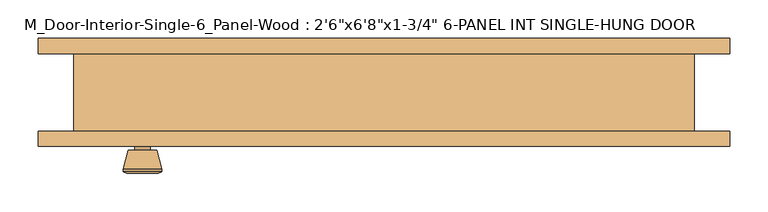
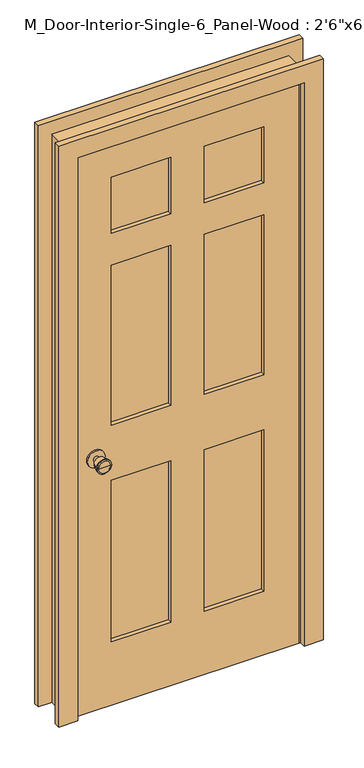
"""IFC4 building model written with IfcOpenShell, lengths in millimetres: door geometry."""

from ifc_helpers import new_model, si_unit, point, frame, frame_2d, origin, place, context, project, spatial, polyline, circle_curve, trimmed, segment, composite_curve, outline, extrude, faceted_brep, source, transform, mapped, element, save
from ifc_brep_helpers import plane_surface, cylinder_surface, revolved_surface, advanced_brep


def door_8e0f4bcc(model_context):
    return source(origin(), model_context, "Body", "SolidModel", [
        advanced_brep(
        [(-316.0, 2.825, 914.4), (-326.0, 2.825, 914.4), (-306.0, 2.825, 914.4), (-295.5241324, 51.825, 914.4), (-336.4758676, 51.825, 914.4), (-316.0, 51.825, 914.4), (-291.0, 49.9971319, 914.4), (-341.0, 49.9971319, 914.4), (-291.0, 46.5334537, 914.4), (-341.0, 46.5334537, 914.4), (-297.363764, 21.825, 914.4), (-334.636236, 21.825, 914.4), (-306.0, 21.825, 914.4), (-326.0, 21.825, 914.4)],
        [
            (0, 1),
            (1, 2, circle_curve(frame((-316.0, 2.825, 914.4), z_axis=(0.0, -1.0, 0.0), x_axis=(-1.0, 0.0, 0.0)), 10.0)),
            (2, 0),
            (2, 1, circle_curve(frame((-316.0, 2.825, 914.4), z_axis=(0.0, -1.0, 0.0), x_axis=(-1.0, 0.0, 0.0)), 10.0)),
            (3, 4, circle_curve(frame((-316.0, 51.825, 914.4), z_axis=(0.0, 1.0, 0.0), x_axis=(-1.0, 0.0, 0.0)), 20.4758676)),
            (4, 5),
            (5, 3),
            (4, 3, circle_curve(frame((-316.0, 51.825, 914.4), z_axis=(0.0, 1.0, 0.0), x_axis=(-1.0, 0.0, 0.0)), 20.4758676)),
            (6, 7, circle_curve(frame((-316.0, 49.9971319, 914.4), z_axis=(0.0, 1.0, 0.0), x_axis=(-1.0, 0.0, 0.0)), 25.0)),
            (7, 4),
            (3, 6),
            (7, 6, circle_curve(frame((-316.0, 49.9971319, 914.4), z_axis=(0.0, 1.0, 0.0), x_axis=(-1.0, 0.0, 0.0)), 25.0)),
            (8, 9, circle_curve(frame((-316.0, 46.5334537, 914.4), z_axis=(0.0, 1.0, 0.0), x_axis=(-1.0, 0.0, 0.0)), 25.0)),
            (9, 7),
            (6, 8),
            (9, 8, circle_curve(frame((-316.0, 46.5334537, 914.4), z_axis=(0.0, 1.0, 0.0), x_axis=(-1.0, 0.0, 0.0)), 25.0)),
            (10, 11, circle_curve(frame((-316.0, 21.825, 914.4), z_axis=(0.0, 1.0, 0.0), x_axis=(-1.0, 0.0, 0.0)), 18.636236)),
            (11, 9),
            (8, 10),
            (11, 10, circle_curve(frame((-316.0, 21.825, 914.4), z_axis=(0.0, 1.0, 0.0), x_axis=(-1.0, 0.0, 0.0)), 18.636236)),
            (12, 13, circle_curve(frame((-316.0, 21.825, 914.4), z_axis=(0.0, 1.0, 0.0), x_axis=(-1.0, 0.0, 0.0)), 10.0)),
            (13, 11),
            (10, 12),
            (13, 12, circle_curve(frame((-316.0, 21.825, 914.4), z_axis=(0.0, 1.0, 0.0), x_axis=(-1.0, 0.0, 0.0)), 10.0)),
            (1, 13),
            (12, 2),
        ],
        [
            plane_surface(frame((-316.0, 2.825, 914.4), z_axis=(0.0, -1.0, 0.0), x_axis=(-1.0, 0.0, 0.0))),
            plane_surface(frame((-316.0, 51.825, 914.4), z_axis=(0.0, 1.0, 0.0), x_axis=(-1.0, 0.0, 0.0))),
            revolved_surface(polyline([(-336.4758676, 51.825, 914.4), (-341.0, 49.9971319, 914.4)]), (-316.0, 2.825, 914.4), (0.0, -1.0, 0.0)),
            cylinder_surface(frame((-316.0, 2.825, 914.4), z_axis=(0.0, -1.0, 0.0), x_axis=(-1.0, 0.0, 0.0)), 25.0),
            revolved_surface(polyline([(-341.0, 46.5334537, 914.4), (-334.636236, 21.825, 914.4)]), (-316.0, 2.825, 914.4), (0.0, -1.0, 0.0)),
            plane_surface(frame((-316.0, 21.825, 914.4), z_axis=(0.0, -1.0, 0.0), x_axis=(-1.0, 0.0, 0.0))),
            cylinder_surface(frame((-316.0, 2.825, 914.4), z_axis=(0.0, -1.0, 0.0), x_axis=(-1.0, 0.0, 0.0)), 10.0),
        ],
        [
            (0, [[1, 2, 3]]),
            (0, [[-3, 4, -1]]),
            (1, [[5, 6, 7]]),
            (1, [[8, -7, -6]]),
            (2, [[9, 10, -5, 11]]),
            (2, [[12, -11, -8, -10]]),
            (3, [[13, 14, -9, 15]]),
            (3, [[16, -15, -12, -14]]),
            (4, [[17, 18, -13, 19]]),
            (4, [[20, -19, -16, -18]]),
            (5, [[21, 22, -17, 23]]),
            (5, [[24, -23, -20, -22]]),
            (6, [[-2, 25, -21, 26]]),
            (6, [[-4, -26, -24, -25]]),
        ],
    ),
        extrude(outline(composite_curve([segment(trimmed(circle_curve(frame_2d((914.4, -316.0)), 30.0), [point((914.4, -346.0))], [point((914.4, -286.0))], False, "CARTESIAN"), True, "CONTINUOUS"), segment(trimmed(circle_curve(frame_2d((914.4, -316.0)), 30.0), [point((914.4, -286.0))], [point((914.4, -346.0))], False, "CARTESIAN"), True, "CONTINUOUS")], self_intersect=False)), frame((0.0, -3.175, 0.0), z_axis=(0.0, 1.0, 0.0), x_axis=(0.0, 0.0, 1.0)), (0.0, 0.0, 1.0), 6.0),
        advanced_brep(
        [(-316.0, -53.625, 914.4), (-306.0, -53.625, 914.4), (-326.0, -53.625, 914.4), (-295.5241324, -102.625, 914.4), (-316.0, -102.625, 914.4), (-336.4758676, -102.625, 914.4), (-291.0, -100.7971319, 914.4), (-341.0, -100.7971319, 914.4), (-291.0, -97.3334537, 914.4), (-341.0, -97.3334537, 914.4), (-297.363764, -72.625, 914.4), (-334.636236, -72.625, 914.4), (-306.0, -72.625, 914.4), (-326.0, -72.625, 914.4)],
        [
            (0, 1),
            (1, 2, circle_curve(frame((-316.0, -53.625, 914.4), z_axis=(0.0, 1.0, 0.0), x_axis=(-1.0, 0.0, 0.0)), 10.0)),
            (2, 0),
            (2, 1, circle_curve(frame((-316.0, -53.625, 914.4), z_axis=(0.0, 1.0, 0.0), x_axis=(-1.0, 0.0, 0.0)), 10.0)),
            (3, 4),
            (4, 5),
            (5, 3, circle_curve(frame((-316.0, -102.625, 914.4), z_axis=(0.0, -1.0, 0.0), x_axis=(-1.0, 0.0, 0.0)), 20.4758676)),
            (3, 5, circle_curve(frame((-316.0, -102.625, 914.4), z_axis=(0.0, -1.0, 0.0), x_axis=(-1.0, 0.0, 0.0)), 20.4758676)),
            (6, 3),
            (5, 7),
            (7, 6, circle_curve(frame((-316.0, -100.7971319, 914.4), z_axis=(0.0, -1.0, 0.0), x_axis=(-1.0, 0.0, 0.0)), 25.0)),
            (6, 7, circle_curve(frame((-316.0, -100.7971319, 914.4), z_axis=(0.0, -1.0, 0.0), x_axis=(-1.0, 0.0, 0.0)), 25.0)),
            (8, 6),
            (7, 9),
            (9, 8, circle_curve(frame((-316.0, -97.3334537, 914.4), z_axis=(0.0, -1.0, 0.0), x_axis=(-1.0, 0.0, 0.0)), 25.0)),
            (8, 9, circle_curve(frame((-316.0, -97.3334537, 914.4), z_axis=(0.0, -1.0, 0.0), x_axis=(-1.0, 0.0, 0.0)), 25.0)),
            (10, 8),
            (9, 11),
            (11, 10, circle_curve(frame((-316.0, -72.625, 914.4), z_axis=(0.0, -1.0, 0.0), x_axis=(-1.0, 0.0, 0.0)), 18.636236)),
            (10, 11, circle_curve(frame((-316.0, -72.625, 914.4), z_axis=(0.0, -1.0, 0.0), x_axis=(-1.0, 0.0, 0.0)), 18.636236)),
            (12, 10),
            (11, 13),
            (13, 12, circle_curve(frame((-316.0, -72.625, 914.4), z_axis=(0.0, -1.0, 0.0), x_axis=(-1.0, 0.0, 0.0)), 10.0)),
            (12, 13, circle_curve(frame((-316.0, -72.625, 914.4), z_axis=(0.0, -1.0, 0.0), x_axis=(-1.0, 0.0, 0.0)), 10.0)),
            (1, 12),
            (13, 2),
        ],
        [
            plane_surface(frame((-316.0, -53.625, 914.4), z_axis=(0.0, 1.0, 0.0), x_axis=(-1.0, 0.0, 0.0))),
            plane_surface(frame((-316.0, -102.625, 914.4), z_axis=(0.0, -1.0, 0.0), x_axis=(-1.0, 0.0, 0.0))),
            revolved_surface(polyline([(-336.4758676, -102.625, 914.4), (-341.0, -100.7971319, 914.4)]), (-316.0, -53.625, 914.4), (0.0, 1.0, 0.0)),
            cylinder_surface(frame((-316.0, -53.625, 914.4), z_axis=(0.0, 1.0, 0.0), x_axis=(-1.0, 0.0, 0.0)), 25.0),
            revolved_surface(polyline([(-341.0, -97.3334537, 914.4), (-334.636236, -72.625, 914.4)]), (-316.0, -53.625, 914.4), (0.0, 1.0, 0.0)),
            plane_surface(frame((-316.0, -72.625, 914.4), z_axis=(0.0, 1.0, 0.0), x_axis=(-1.0, 0.0, 0.0))),
            cylinder_surface(frame((-316.0, -53.625, 914.4), z_axis=(0.0, 1.0, 0.0), x_axis=(-1.0, 0.0, 0.0)), 10.0),
        ],
        [
            (0, [[1, 2, 3]]),
            (0, [[-3, 4, -1]]),
            (1, [[5, 6, 7]]),
            (1, [[-6, -5, 8]]),
            (2, [[9, -7, 10, 11]]),
            (2, [[-10, -8, -9, 12]]),
            (3, [[13, -11, 14, 15]]),
            (3, [[-14, -12, -13, 16]]),
            (4, [[17, -15, 18, 19]]),
            (4, [[-18, -16, -17, 20]]),
            (5, [[21, -19, 22, 23]]),
            (5, [[-22, -20, -21, 24]]),
            (6, [[25, -23, 26, -2]]),
            (6, [[-26, -24, -25, -4]]),
        ],
    ),
        extrude(outline(composite_curve([segment(trimmed(circle_curve(frame_2d((914.4, -316.0)), 30.0), [point((914.4, -346.0))], [point((914.4, -286.0))], False, "CARTESIAN"), True, "CONTINUOUS"), segment(trimmed(circle_curve(frame_2d((914.4, -316.0)), 30.0), [point((914.4, -286.0))], [point((914.4, -346.0))], False, "CARTESIAN"), True, "CONTINUOUS")], self_intersect=False)), frame((0.0, -53.625, 0.0), z_axis=(0.0, 1.0, 0.0), x_axis=(0.0, 0.0, 1.0)), (0.0, 0.0, 1.0), 6.0),
        extrude(outline(polyline([(261.0, -17.9916667), (261.0, -32.8083333), (57.5, -32.8083333), (57.5, -17.9916667), (261.0, -17.9916667)])), frame((0.0, 0.0, 1708.5), z_axis=(0.0, 0.0, 1.0), x_axis=(1.0, 0.0, 0.0)), (0.0, 0.0, 1.0), 203.5),
        extrude(outline(polyline([(261.0, -17.9916667), (261.0, -32.8083333), (57.5, -32.8083333), (57.5, -17.9916667), (261.0, -17.9916667)])), frame((0.0, 0.0, 1014.4), z_axis=(0.0, 0.0, 1.0), x_axis=(1.0, 0.0, 0.0)), (0.0, 0.0, 1.0), 579.1),
        extrude(outline(polyline([(-57.5, -17.9916667), (-57.5, -32.8083333), (-261.0, -32.8083333), (-261.0, -17.9916667), (-57.5, -17.9916667)])), frame((0.0, 0.0, 1014.4), z_axis=(0.0, 0.0, 1.0), x_axis=(1.0, 0.0, 0.0)), (0.0, 0.0, 1.0), 579.1),
        extrude(outline(polyline([(-57.5, -17.9916667), (-57.5, -32.8083333), (-261.0, -32.8083333), (-261.0, -17.9916667), (-57.5, -17.9916667)])), frame((0.0, 0.0, 1708.5), z_axis=(0.0, 0.0, 1.0), x_axis=(1.0, 0.0, 0.0)), (0.0, 0.0, 1.0), 203.5),
        extrude(outline(polyline([(261.0, -17.9916667), (261.0, -32.8083333), (57.5, -32.8083333), (57.5, -17.9916667), (261.0, -17.9916667)])), frame((0.0, 0.0, 230.0), z_axis=(0.0, 0.0, 1.0), x_axis=(1.0, 0.0, 0.0)), (0.0, 0.0, 1.0), 584.4),
        extrude(outline(polyline([(-57.5, -17.9916667), (-57.5, -32.8083333), (-261.0, -32.8083333), (-261.0, -17.9916667), (-57.5, -17.9916667)])), frame((0.0, 0.0, 230.0), z_axis=(0.0, 0.0, 1.0), x_axis=(1.0, 0.0, 0.0)), (0.0, 0.0, 1.0), 584.4),
        extrude(outline(polyline([(2032.0, -381.0), (0.0, -381.0), (0.0, 381.0), (2032.0, 381.0), (2032.0, -381.0)]), holes=[polyline([(1912.0, 57.5), (1912.0, 261.0), (1708.5, 261.0), (1708.5, 57.5), (1912.0, 57.5)]), polyline([(1593.5, 261.0), (1014.4, 261.0), (1014.4, 57.5), (1593.5, 57.5), (1593.5, 261.0)]), polyline([(1014.4, -57.5), (1014.4, -261.0), (1593.5, -261.0), (1593.5, -57.5), (1014.4, -57.5)]), polyline([(1708.5, -261.0), (1912.0, -261.0), (1912.0, -57.5), (1708.5, -57.5), (1708.5, -261.0)]), polyline([(814.4, 57.5), (814.4, 261.0), (230.0, 261.0), (230.0, 57.5), (814.4, 57.5)]), polyline([(230.0, -57.5), (230.0, -261.0), (814.4, -261.0), (814.4, -57.5), (230.0, -57.5)])]), frame((0.0, -47.625, 0.0), z_axis=(0.0, 1.0, 0.0), x_axis=(0.0, 0.0, 1.0)), (0.0, 0.0, 1.0), 44.45),
        faceted_brep([(406.0, -47.625, 0.0), (381.0, -47.625, 0.0), (381.0, -3.175, 0.0), (368.3, -3.175, 0.0), (368.3, 31.75, 0.0), (381.0, 31.75, 0.0), (381.0, 53.975, 0.0), (406.0, 53.975, 0.0), (406.0, 53.975, 2057.0), (406.0, -47.625, 2057.0), (381.0, 53.975, 2032.0), (-381.0, 53.975, 2032.0), (-381.0, 53.975, 0.0), (-406.0, 53.975, 0.0), (-406.0, 53.975, 2057.0), (381.0, 31.75, 2032.0), (368.3, 31.75, 2019.3), (-368.3, 31.75, 2019.3), (-368.3, 31.75, 0.0), (-381.0, 31.75, 0.0), (-381.0, 31.75, 2032.0), (368.3, -3.175, 2019.3), (381.0, -3.175, 2032.0), (-381.0, -3.175, 2032.0), (-381.0, -3.175, 0.0), (-368.3, -3.175, 0.0), (-368.3, -3.175, 2019.3), (381.0, -47.625, 2032.0), (-406.0, -47.625, 2057.0), (-406.0, -47.625, 0.0), (-381.0, -47.625, 0.0), (-381.0, -47.625, 2032.0)], [[[0, 1, 2, 3, 4, 5, 6, 7]], [[7, 8, 9, 0]], [[6, 10, 11, 12, 13, 14, 8, 7]], [[5, 15, 10, 6]], [[4, 16, 17, 18, 19, 20, 15, 5]], [[3, 21, 16, 4]], [[2, 22, 23, 24, 25, 26, 21, 3]], [[1, 27, 22, 2]], [[0, 9, 28, 29, 30, 31, 27, 1]], [[8, 14, 28, 9]], [[15, 20, 11, 10]], [[21, 26, 17, 16]], [[27, 31, 23, 22]], [[29, 13, 12, 19, 18, 25, 24, 30]], [[14, 13, 29, 28]], [[20, 19, 12, 11]], [[26, 25, 18, 17]], [[31, 30, 24, 23]]]),
        extrude(outline(polyline([(0.0, 452.35), (2103.35, 452.35), (2103.35, -452.35), (0.0, -452.35), (0.0, -387.35), (2038.35, -387.35), (2038.35, 387.35), (0.0, 387.35), (0.0, 452.35)])), frame((0.0, 53.975, 0.0), z_axis=(0.0, 1.0, 0.0), x_axis=(0.0, 0.0, 1.0)), (0.0, 0.0, 1.0), 20.0),
        extrude(outline(polyline([(0.0, 452.35), (2103.35, 452.35), (2103.35, -452.35), (0.0, -452.35), (0.0, -387.35), (2038.35, -387.35), (2038.35, 387.35), (0.0, 387.35), (0.0, 452.35)])), frame((0.0, -67.625, 0.0), z_axis=(0.0, 1.0, 0.0), x_axis=(0.0, 0.0, 1.0)), (0.0, 0.0, 1.0), 20.0),
    ])


if __name__ == "__main__":
    model = new_model("IFC4")
    model_context = context("Model", 3, world=origin())
    ifc_project = project(units=[si_unit("LENGTHUNIT", "METRE", prefix="MILLI")], contexts=[model_context])
    site = spatial("IfcSite", under=ifc_project)
    building = spatial("IfcBuilding", under=site)
    placement = place(None, origin())
    door_shape = door_8e0f4bcc(model_context)
    element("IfcDoor", 1, ObjectType="M_Door-Interior-Single-6_Panel-Wood : 2'6\"x6'8\"x1-3/4\" 6-PANEL INT SINGLE-HUNG DOOR", at=placement, inside=building, context=model_context, shape_type="MappedRepresentation", body=[
        mapped(door_shape, transform((0.0, 0.0, 0.0), x_axis=(1.0, 0.0, 0.0), y_axis=(0.0, 1.0, 0.0), z_axis=(0.0, 0.0, 1.0))),
    ])
    save(model, "model.ifc")

# Revit data of these elements
# Type "M_Door-Interior-Single-6_Panel-Wood : 2'6\"x6'8\"x1-3/4\" 6-PANEL INT SINGLE-HUNG DOOR"
#   Type Mark = "11"
#   Assembly Code = "C1020300"
#   Analytic Construction = "Wooden"
#   Top Rail = 0' - 4.72441"
#   Top Panel = 0' - 8.01181"
#   Thickness = 0' - 1 3/4"
#   Thermal Resistance (R) = 2.5876 (h·ft²·°F)/BTU
#   Swing Angle [instance default] = 90.00°
#   Stiles = 0' - 4.72441"
#   Rough Width = 2' - 7.9685"
#   Rough Height = 6' - 8.98425"
#   Mullion = 0' - 4.52756"
#   Lock Rail = 0' - 7.87402"
#   Intermediate Rail = 0' - 4.52756"
#   Height = 6' - 8"
#   Width = 2' - 6"
#   Heat Transfer Coefficient (U) = 0.3865 BTU/(h·ft²·°F)
#   Bottom Rail = 0' - 9.05512"
#   Trim Material = Cherry
#   Panel Material = Cherry
#   Frame Material = Cherry
#   Door Handle Material = Aluminum
#   Visual Light Transmittance = 0
#   Solar Heat Gain Coefficient = 0
#   Wall Closure = (empty or 0)
#   Function = (empty or 0)
# Element 1 (IfcDoor, "M_Door-Interior-Single-6_Panel-Wood : 2'6\"x6'8\"x1-3/4\" 6-PANEL INT SINGLE-HUNG DOOR")
#   Materials on its faces: "Cherry", "Aluminum"
# Materials
#   "Cherry": class "Wood", colour RGB 226 177 128, transparency 0, Description = "Prunus Serotina", Cost = 0
#   "Aluminum": class "Metal", colour RGB 244 244 244, transparency 0, Description = "Aluminum 6061", Cost = 0
